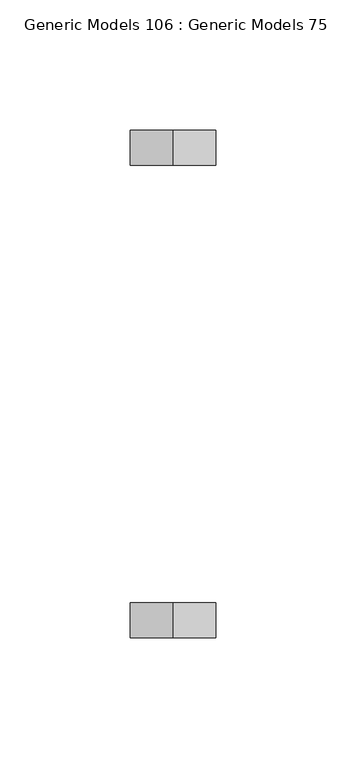
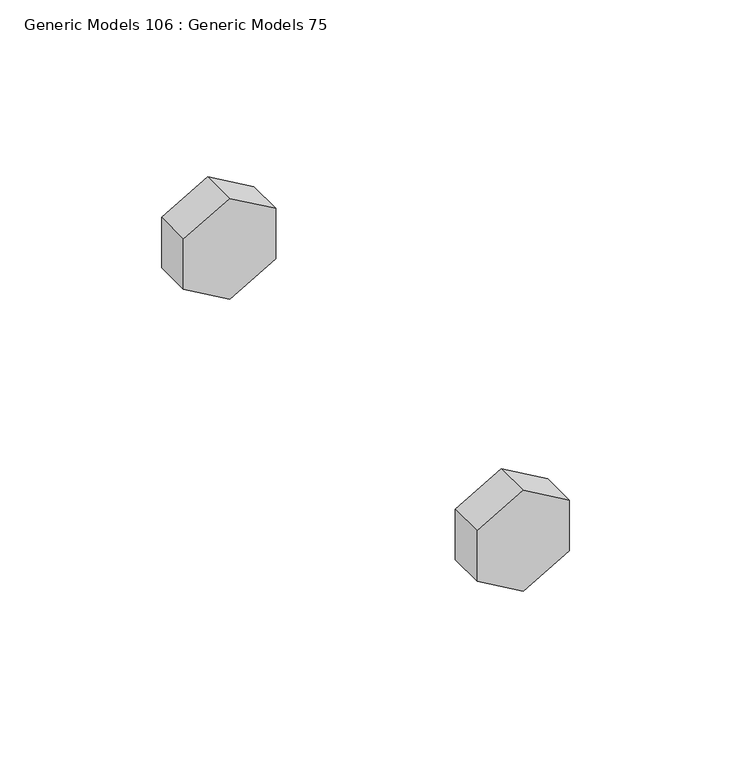
"""IFC4 building model written with IfcOpenShell, lengths in millimetres: proxy geometry, Generic Models 106 : Generic Models 75."""

from ifc_helpers import new_model, si_unit, frame, origin, place, context, project, spatial, polyline, outline, extrude, source, transform, mapped, element, save


def generic_models_106_generic_models_75_9af4e480(model_context):
    return source(origin(), model_context, "Body", "SweptSolid", [
        extrude(outline(polyline([(266616.6501684, 31991.9073871), (266635.7001684, 31991.9073871), (266645.2251684, 31975.4096032), (266635.7001684, 31958.9118192), (266616.6501684, 31958.9118192), (266607.1251684, 31975.4096032), (266616.6501684, 31991.9073871)])), frame((0.0, 30858.4781612, 0.0), z_axis=(0.0, 1.0, 0.0), x_axis=(0.0, 0.0, 1.0)), (0.0, 0.0, 1.0), 13.49375),
        extrude(outline(polyline([(266616.6501684, 31991.9073871), (266635.7001684, 31991.9073871), (266645.2251684, 31975.4096032), (266635.7001684, 31958.9118192), (266616.6501684, 31958.9118192), (266607.1251684, 31975.4096032), (266616.6501684, 31991.9073871)])), frame((0.0, 30676.7094112, 0.0), z_axis=(0.0, 1.0, 0.0), x_axis=(0.0, 0.0, 1.0)), (0.0, 0.0, 1.0), 13.49375),
    ])


if __name__ == "__main__":
    model = new_model("IFC4")
    model_context = context("Model", 3, world=origin())
    ifc_project = project(units=[si_unit("LENGTHUNIT", "METRE", prefix="MILLI")], contexts=[model_context])
    site = spatial("IfcSite", under=ifc_project)
    building = spatial("IfcBuilding", under=site)
    placement = place(None, origin())
    generic_models_106_generic_models_75_shape = generic_models_106_generic_models_75_9af4e480(model_context)
    element("IfcBuildingElementProxy", 1, Name="Generic Models 106 : Generic Models 75", ObjectType="Generic Models 106 : Generic Models 75", at=placement, inside=building, context=model_context, shape_type="MappedRepresentation", body=[
        mapped(generic_models_106_generic_models_75_shape, transform((0.0, 0.0, 0.0), x_axis=(1.0, 0.0, 0.0), y_axis=(0.0, 1.0, 0.0), z_axis=(0.0, 0.0, 1.0))),
    ])
    save(model, "model.ifc")
